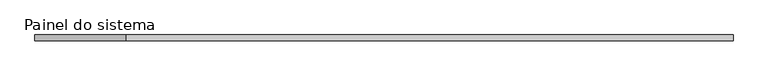
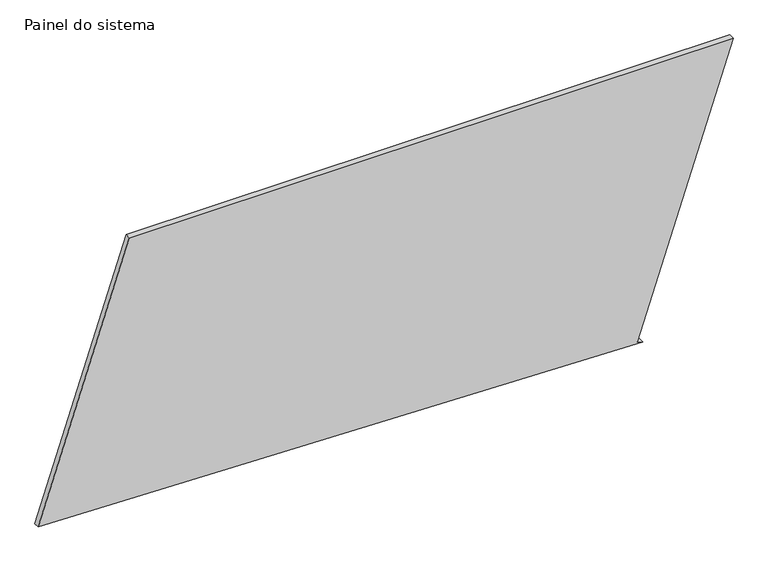
"""IFC4 building model written with IfcOpenShell, lengths in millimetres: plate geometry, Painel do sistema : Envidraçado."""

from ifc_helpers import new_model, si_unit, frame, origin, place, context, project, spatial, polyline, outline, extrude, source, transform, mapped, element, save


def painel_do_sistema_c4f84099(model_context):
    return source(origin(), model_context, "Body", "SweptSolid", [
        extrude(outline(polyline([(0.0, 1142.7479865), (7.8961296, 1119.027718), (1288.1278591, 1545.1980925), (1288.1278591, -1139.8779167), (70.5309056, -1545.1980925), (0.0, 1142.7479865)])), frame((0.0, 24.5, 0.0), z_axis=(0.0, 1.0, 0.0), x_axis=(0.0, 0.0, 1.0)), (0.0, 0.0, 1.0), 25.0),
    ])


if __name__ == "__main__":
    model = new_model("IFC4")
    model_context = context("Model", 3, world=origin())
    ifc_project = project(units=[si_unit("LENGTHUNIT", "METRE", prefix="MILLI")], contexts=[model_context])
    site = spatial("IfcSite", under=ifc_project)
    building = spatial("IfcBuilding", under=site)
    placement = place(None, origin())
    painel_do_sistema_shape = painel_do_sistema_c4f84099(model_context)
    element("IfcPlate", 1, ObjectType="Painel do sistema : Envidraçado", at=placement, inside=building, context=model_context, shape_type="MappedRepresentation", body=[
        mapped(painel_do_sistema_shape, transform((0.0, 0.0, 0.0), x_axis=(1.0, 0.0, 0.0), y_axis=(0.0, 1.0, 0.0), z_axis=(0.0, 0.0, 1.0))),
    ])
    save(model, "model.ifc")

# Revit data of these elements
# Type "Painel do sistema : Envidraçado"
#   Construction Type Id = "GSP4R"
#   Analytic Construction = "Vidraça única Pilkington 1/8 pol"
#   Visual Light Transmittance = 0.9
#   Solar Heat Gain Coefficient = 0.86
#   Heat Transfer Coefficient (U) = 6.7069 W/(m²·K)
# Element 1 (IfcPlate, "Painel do sistema : Envidraçado")
#   Materials on its faces: "Vidro"
# Materials
#   "Vidro": class "Vidro", colour RGB 0 128 192, transparency 0.9, Description = "Vidro de sílica", Cost = 0
